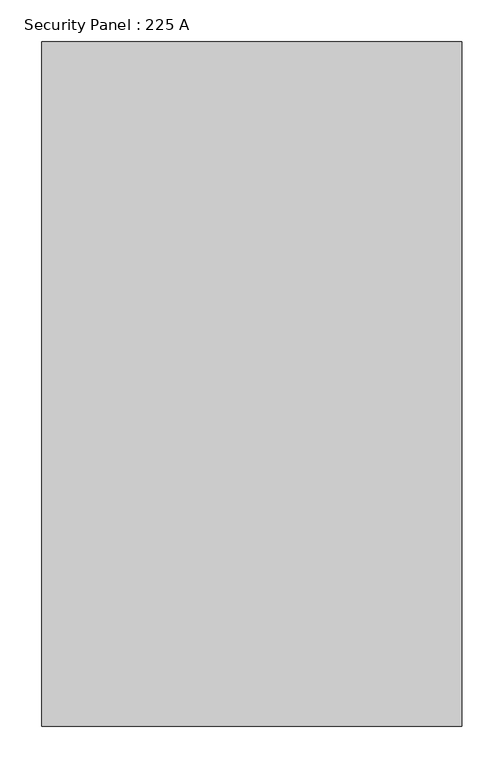
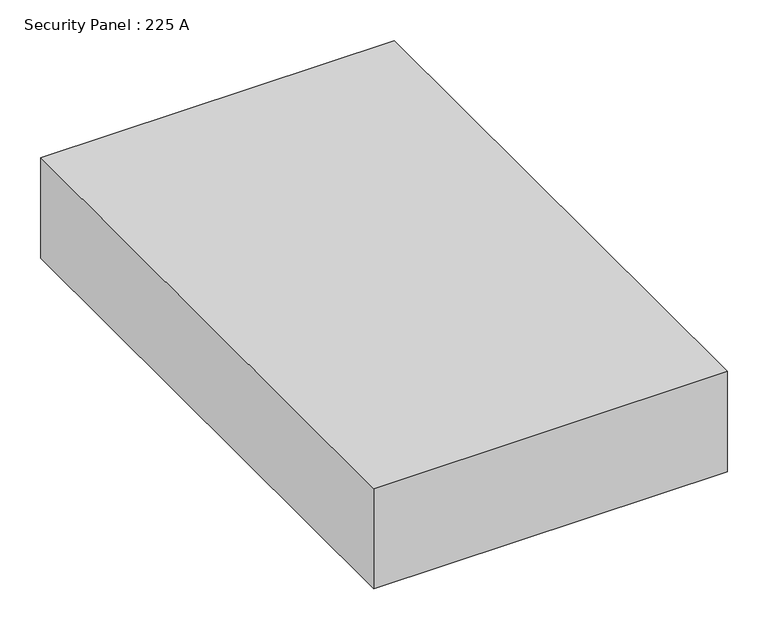
"""IFC4 building model written with IfcOpenShell, lengths in millimetres: proxy geometry, Security Panel : 225 A."""

from ifc_helpers import new_model, si_unit, frame, origin, place, context, project, spatial, polyline, outline, extrude, source, transform, mapped, element, save


def security_panel_225_a_071659d5(model_context):
    return source(origin(), model_context, "Body", "SweptSolid", [
        extrude(outline(polyline([(250.0, -11.6), (250.0, -826.6), (-250.0, -826.6), (-250.0, -11.6), (250.0, -11.6)])), frame((0.0, 0.0, -150.0), z_axis=(0.0, 0.0, 1.0), x_axis=(1.0, 0.0, 0.0)), (0.0, 0.0, 1.0), 150.0),
    ])


if __name__ == "__main__":
    model = new_model("IFC4")
    model_context = context("Model", 3, world=origin())
    ifc_project = project(units=[si_unit("LENGTHUNIT", "METRE", prefix="MILLI")], contexts=[model_context])
    site = spatial("IfcSite", under=ifc_project)
    building = spatial("IfcBuilding", under=site)
    placement = place(None, origin())
    security_panel_225_a_shape = security_panel_225_a_071659d5(model_context)
    element("IfcBuildingElementProxy", 1, Name="Security Panel : 225 A", ObjectType="Security Panel : 225 A", at=placement, inside=building, context=model_context, shape_type="MappedRepresentation", body=[
        mapped(security_panel_225_a_shape, transform((0.0, 0.0, 0.0), x_axis=(1.0, 0.0, 0.0), y_axis=(0.0, 1.0, 0.0), z_axis=(0.0, 0.0, 1.0))),
    ])
    save(model, "model.ifc")

# Revit data of these elements
# Type "Security Panel : 225 A"
#   Type Mark = "Security Panel"
#   Classification.OmniClass.21.Number = "21-04 70 10 50"
#   Classification.MasterFormat.Description = "Electronic Access Control and Intrusion Detection"
#   Classification.OmniClass.21.Description = "Intruction Detection"
#   Classification.UniFormat.II.Description = "Intruction Detection"
#   Classification.MasterFormat.Number = "28 10 00"
#   Classification.OmniClass.23.Number = "23-35 31 29"
#   Classification.OmniClass.23.Description = "Switchboards"
#   Classification.UniFormat.II.Number = "D7010.50"
#   COBie.Type.CreatedBy = "info@mma.ie"
#   COBie.Type.CreatedOn = "2017-07-26T09:12:43"
#   COBie.Type.Name = "Security Panel"
#   COBie.Type.Category = "23-35 31 29 : Switchboards"
#   COBie.Type.Description = "Security Panel_225 A"
#   COBie.Type.AssetType = "Fixed"
#   COBie.Type.Manufacturer = ""
#   COBie.Type.ModelNumber = ""
#   built-in parameter 1140081 [instance default] = "Recessed"
#   Keynote = "26 24 16.A"
#   built-in parameter 1140083 [instance default] = "Type 1"
#   COBie.Type.ReplacementCost = 0
#   Width = 508 mm
#   SP-Width = 500 mm
#   SP-Height = 815 mm
#   SP-Depth = 150 mm
#   built-in parameter 1140082 [instance default] = 100 (stored number, unit not read)
#   built-in parameter 1140140 [instance default] = 1 (stored number, unit not read)
#   Height [instance default] = 812.8 mm
#   Depth = 146.1 mm
#   Default Elevation = 1200 mm
#   42 Circuit Height = 1041.4 mm
#   30 Circuit Height = 812.8 mm
#   24 Circuit Height = 812.8 mm
#   12 Circuit Height = 812.8 mm
#   COBie.Type = yes
#   built-in parameter 1140142 [instance default] = -1
#   built-in parameter 1140079 [instance default] = 12
#   built-in parameter 1155100 [instance default] = -1
#   Load Classification = Other
